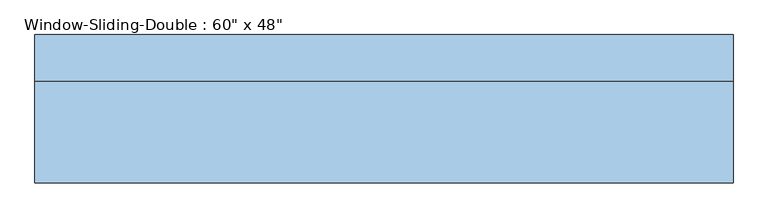
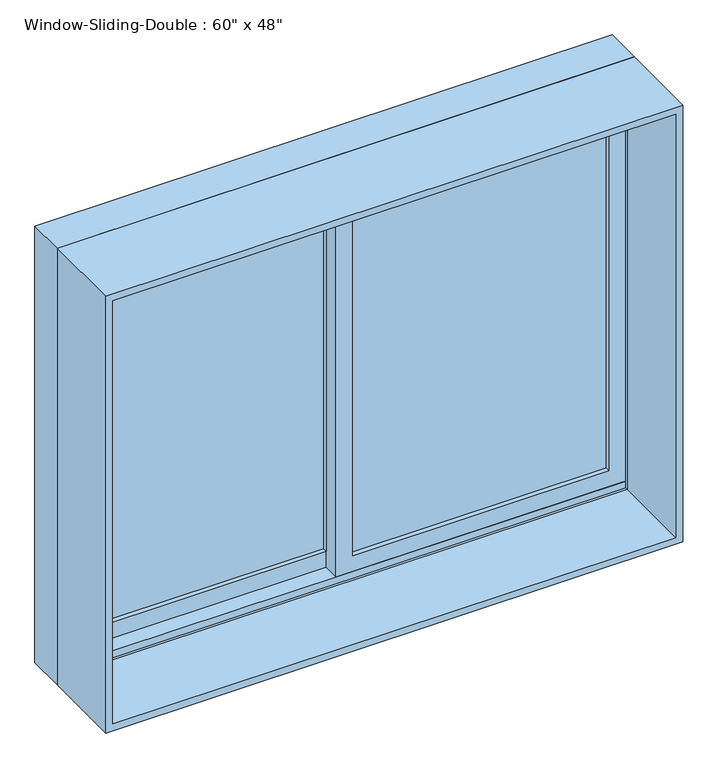
"""IFC4 building model written with IfcOpenShell, lengths in millimetres: window geometry."""

from ifc_helpers import new_model, si_unit, frame, origin, place, context, project, spatial, polyline, outline, extrude, faceted_brep, source, transform, mapped, element, save


def window_eb22a4a1(model_context):
    return source(origin(), model_context, "Body", "SolidModel", [
        faceted_brep([(-762.0, 66.04, 914.4), (-762.0, 167.64, 914.4), (762.0, 167.64, 914.4), (762.0, 66.04, 914.4), (-721.0778905, 167.64, 2092.6778905), (-721.0778905, 161.29, 2092.6778905), (-721.0778905, 161.29, 933.45), (-721.0778905, 167.64, 933.45), (721.0778905, 161.29, 2092.6778905), (721.0778905, 161.29, 933.45), (742.95, 161.29, 933.45), (742.95, 161.29, 2114.55), (-742.95, 161.29, 2114.55), (-742.95, 161.29, 933.45), (-742.95, 66.04, 2114.55), (-742.95, 66.04, 933.45), (-742.95, 72.39, 933.45), (-742.95, 72.39, 952.5), (-742.95, 116.84, 952.5), (-742.95, 116.84, 933.45), (762.0, 66.04, 2133.6), (-762.0, 66.04, 2133.6), (742.95, 66.04, 2114.55), (742.95, 66.04, 933.45), (-762.0, 167.64, 2133.6), (762.0, 167.64, 2133.6), (721.0778905, 167.64, 933.45), (721.0778905, 167.64, 2092.6778905), (742.95, 116.84, 933.45), (742.95, 116.84, 952.5), (742.95, 72.39, 952.5), (742.95, 72.39, 933.45)], [[[0, 1, 2, 3]], [[4, 5, 6, 7]], [[5, 8, 9, 10, 11, 12, 13, 6]], [[12, 14, 15, 16, 17, 18, 19, 13]], [[0, 3, 20, 21], [22, 23, 15, 14]], [[24, 1, 0, 21]], [[2, 1, 24, 25], [4, 7, 26, 27]], [[5, 4, 27, 8]], [[12, 11, 22, 14]], [[21, 20, 25, 24]], [[8, 27, 26, 9]], [[22, 11, 10, 28, 29, 30, 31, 23]], [[20, 3, 2, 25]], [[26, 7, 6, 13, 19, 28, 10, 9]], [[28, 19, 18, 29]], [[29, 18, 17, 30]], [[30, 17, 16, 31]], [[15, 23, 31, 16]]]),
        extrude(outline(polyline([(2133.6, -762.0), (914.4, -762.0), (914.4, 762.0), (2133.6, 762.0), (2133.6, -762.0)]), holes=[polyline([(2114.55, 742.95), (933.45, 742.95), (933.45, -742.95), (2114.55, -742.95), (2114.55, 742.95)])]), frame((0.0, -156.21, 0.0), z_axis=(0.0, 1.0, 0.0), x_axis=(0.0, 0.0, 1.0)), (0.0, 0.0, 1.0), 222.25),
        extrude(outline(polyline([(698.5, 104.14), (698.5, 97.79), (22.225, 97.79), (22.225, 104.14), (698.5, 104.14)])), frame((0.0, 0.0, 996.95), z_axis=(0.0, 0.0, 1.0), x_axis=(1.0, 0.0, 0.0)), (0.0, 0.0, 1.0), 1073.15),
        extrude(outline(polyline([(698.5, 91.44), (698.5, 85.09), (22.225, 85.09), (22.225, 91.44), (698.5, 91.44)])), frame((0.0, 0.0, 996.95), z_axis=(0.0, 0.0, 1.0), x_axis=(1.0, 0.0, 0.0)), (0.0, 0.0, 1.0), 1073.15),
        extrude(outline(polyline([(-22.225, 148.59), (-22.225, 142.24), (-698.5, 142.24), (-698.5, 148.59), (-22.225, 148.59)])), frame((0.0, 0.0, 996.95), z_axis=(0.0, 0.0, 1.0), x_axis=(1.0, 0.0, 0.0)), (0.0, 0.0, 1.0), 1073.15),
        extrude(outline(polyline([(-22.225, 135.89), (-22.225, 129.54), (-698.5, 129.54), (-698.5, 135.89), (-22.225, 135.89)])), frame((0.0, 0.0, 996.95), z_axis=(0.0, 0.0, 1.0), x_axis=(1.0, 0.0, 0.0)), (0.0, 0.0, 1.0), 1073.15),
        extrude(outline(polyline([(933.45, -742.95), (933.45, 22.225), (2114.55, 22.225), (2114.55, -742.95), (933.45, -742.95)]), holes=[polyline([(2070.1, -22.225), (996.95, -22.225), (996.95, -698.5), (2070.1, -698.5), (2070.1, -22.225)])]), frame((0.0, 116.84, 0.0), z_axis=(0.0, 1.0, 0.0), x_axis=(0.0, 0.0, 1.0)), (0.0, 0.0, 1.0), 44.45),
        extrude(outline(polyline([(952.5, 742.95), (2114.55, 742.95), (2114.55, -22.225), (952.5, -22.225), (952.5, 742.95)]), holes=[polyline([(996.95, 22.225), (2070.1, 22.225), (2070.1, 698.5), (996.95, 698.5), (996.95, 22.225)])]), frame((0.0, 72.39, 0.0), z_axis=(0.0, 1.0, 0.0), x_axis=(0.0, 0.0, 1.0)), (0.0, 0.0, 1.0), 44.45),
    ])


if __name__ == "__main__":
    model = new_model("IFC4")
    model_context = context("Model", 3, world=origin())
    ifc_project = project(units=[si_unit("LENGTHUNIT", "METRE", prefix="MILLI")], contexts=[model_context])
    site = spatial("IfcSite", under=ifc_project)
    building = spatial("IfcBuilding", under=site)
    placement = place(None, origin())
    window_shape = window_eb22a4a1(model_context)
    element("IfcWindow", 1, ObjectType="Window-Sliding-Double : 60\" x 48\"", at=placement, inside=building, context=model_context, shape_type="MappedRepresentation", body=[
        mapped(window_shape, transform((0.0, 0.0, 0.0), x_axis=(1.0, 0.0, 0.0), y_axis=(0.0, 1.0, 0.0), z_axis=(0.0, 0.0, 1.0))),
    ])
    save(model, "model.ifc")

# Revit data of these elements
# Type "Window-Sliding-Double : 60\" x 48\""
#   Type Mark = "A"
#   Fire Rating = "0.5h"
#   Assembly Code = "B2020100"
#   Analytic Construction = "Double glazing - domestic"
#   Window Inset [instance default] = 0' - 0"
#   Wall Thickness [instance default] = 0' - 6"
#   Visual Light Transmittance = 0.81
#   Thermal Resistance (R) = 1.8146 (h·ft²·°F)/BTU
#   Solar Heat Gain Coefficient = 0.76
#   Muntin Width = 2' - 2 5/8"
#   Muntin Height = 3' - 6 1/4"
#   Interior Wall Closure [instance default] = 0' - 2 3/4"
#   Heat Transfer Coefficient (U) = 0.5511 BTU/(h·ft²·°F)
#   Frame Extension [instance default] = 0' - 0 1/4"
#   Exterior Wall Closure [instance default] = 0' - 1 1/4"
#   Rough Width = 5' - 0 1/2"
#   Rough Height = 4' - 0 1/2"
#   Height = 4' - 0"
#   Extension Jamb [instance default] = 0' - 2 3/4"
#   Default Sill Height = 3' - 0"
#   Width = 5' - 0"
#   Interior Trim Visibility [instance default] = yes
#   Indicator Visibility [instance default] = yes
#   Exterior Trim Visibility [instance default] = yes
#   Muntin Visibility = yes
#   Extension Jamb Visibility [instance default] = yes
#   Muntin Pattern = Muntin Pattern_2x2 : Muntin Pattern_2x2
#   Interior Trim Material = Cherry
#   Interior Trim = Trim-Window-Interior-Flat : Picture Frame
#   Interior Frame Material = Cherry
#   Glass Panel Material = Glass, Clear Glazing
#   Exterior Trim Material = PVC, Flexible
#   Exterior Trim = Trim-Window-Exterior-Flat : with Sill
#   Exterior Frame Material = PVC, Flexible
#   Wall Closure = (empty or 0)
# Element 1 (IfcWindow, "Window-Sliding-Double : 60\" x 48\"")
#   Wall Thickness = 1' - 0"
#   Extension Jamb = 0' - 8 3/4"
#   Materials on its faces: "Cherry", "Glass, Clear Glazing", "PVC, Flexible"
# Materials
#   "Cherry": class "Wood", colour RGB 157 77 38, transparency 0, Description = "Prunus Serotina", Cost = 0
#   "Glass, Clear Glazing": class "Glass", colour RGB 120 120 120, transparency 0, Description = "Clear glazing", Cost = 0
#   "PVC, Flexible": class "Plastic", colour RGB 178 178 178, transparency 0, Description = "Flexible polyvinyl chloride", Cost = 0
